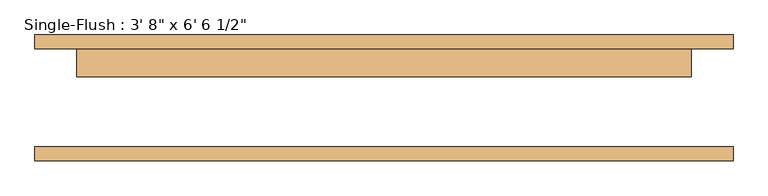
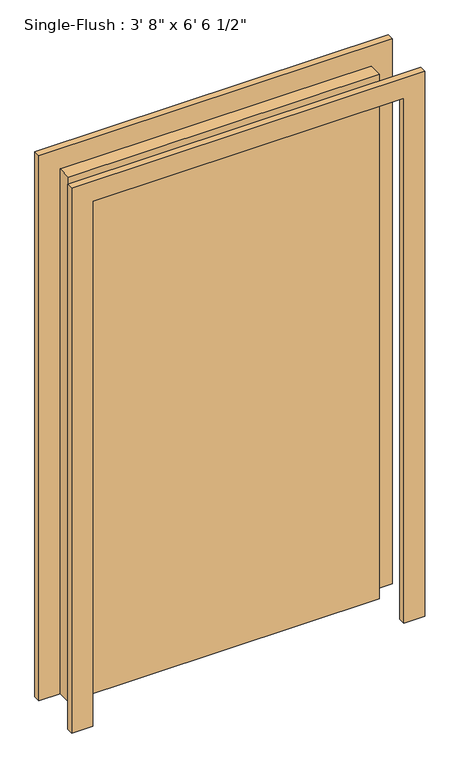
"""IFC4 building model written with IfcOpenShell, lengths in millimetres: door geometry."""

from ifc_helpers import new_model, si_unit, frame, origin, origin_with_axes, place, context, project, spatial, polyline, outline, extrude, source, transform, mapped, element, save


def door_7f50078a(model_context):
    return source(origin(), model_context, "Body", "SweptSolid", [
        extrude(outline(polyline([(2070.1, -635.0), (0.0, -635.0), (0.0, -558.8), (1993.9, -558.8), (1993.9, 558.8), (0.0, 558.8), (0.0, 635.0), (2070.1, 635.0), (2070.1, -635.0)])), frame((0.0, 88.9, 0.0), z_axis=(0.0, 1.0, 0.0), x_axis=(0.0, 0.0, 1.0)), (0.0, 0.0, 1.0), 25.4),
        extrude(outline(polyline([(2070.1, 635.0), (2070.1, -635.0), (0.0, -635.0), (0.0, -558.8), (1993.9, -558.8), (1993.9, 558.8), (0.0, 558.8), (0.0, 635.0), (2070.1, 635.0)])), frame((0.0, -114.3, 0.0), z_axis=(0.0, 1.0, 0.0), x_axis=(0.0, 0.0, 1.0)), (0.0, 0.0, 1.0), 25.4),
        extrude(outline(polyline([(558.8, 38.1), (-558.8, 38.1), (-558.8, 88.9), (558.8, 88.9), (558.8, 38.1)])), origin_with_axes(), (0.0, 0.0, 1.0), 1993.9),
    ])


if __name__ == "__main__":
    model = new_model("IFC4")
    model_context = context("Model", 3, world=origin())
    ifc_project = project(units=[si_unit("LENGTHUNIT", "METRE", prefix="MILLI")], contexts=[model_context])
    site = spatial("IfcSite", under=ifc_project)
    building = spatial("IfcBuilding", under=site)
    placement = place(None, origin())
    door_shape = door_7f50078a(model_context)
    element("IfcDoor", 1, ObjectType="Single-Flush : 3' 8\" x 6' 6 1/2\"", at=placement, inside=building, context=model_context, shape_type="MappedRepresentation", body=[
        mapped(door_shape, transform((0.0, 0.0, 0.0), x_axis=(1.0, 0.0, 0.0), y_axis=(0.0, 1.0, 0.0), z_axis=(0.0, 0.0, 1.0))),
    ])
    save(model, "model.ifc")

# Revit data of these elements
# Type "Single-Flush : 3' 8\" x 6' 6 1/2\""
#   Type Mark = "10"
#   Assembly Code = "C1020"
#   Thickness = 0' - 2"
#   Height = 6' - 6 1/2"
#   Trim Projection Ext = 0' - 1"
#   Trim Projection Int = 0' - 1"
#   Trim Width = 0' - 3"
#   Width = 3' - 8"
#   Door Material = Door - Panel
#   Frame Material = Door - Frame
#   Function = (empty or 0)
#   Wall Closure = (empty or 0)
# Element 1 (IfcDoor, "Single-Flush : 3' 8\" x 6' 6 1/2\"")
#   Materials on its faces: "Door - Frame", "Door - Panel"
# Materials
#   "Door - Panel": class "Wood", colour RGB 114 82 51, transparency 0
#   "Door - Frame": class "Miscellaneous", colour RGB 153 76 43, transparency 0
